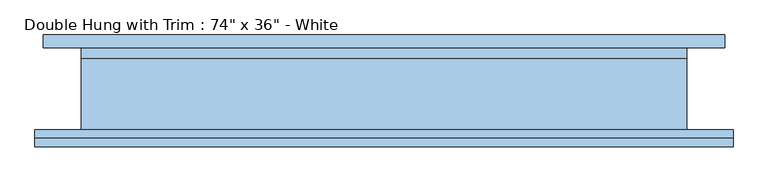
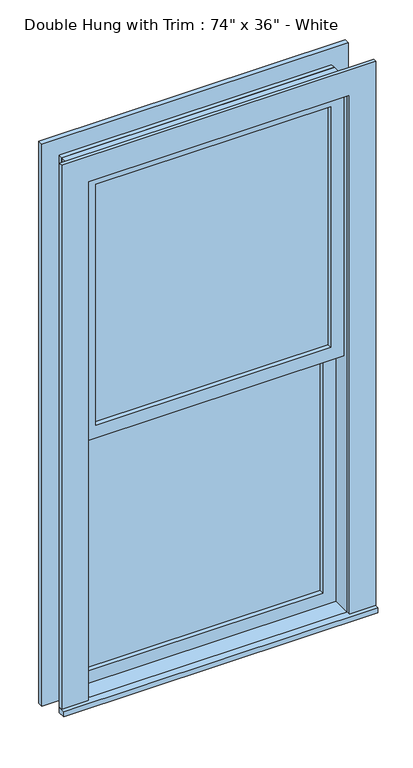
"""IFC4 building model written with IfcOpenShell, lengths in millimetres: window geometry."""

import ifcopenshell
import ifcopenshell.guid

model = None  # the IFC model being written
_history = None  # IfcOwnerHistory: only IFC2X3 demands one
_inside = {}  # id of a spatial element -> (the spatial element, [elements in it])
_under = {}  # id of a project, library or spatial element -> (it, [spatial elements below it])
_declared = {}  # id of a project -> (the project, [libraries it declares])
_typed = {}  # id of a type object -> (the type object, [elements of that type])
_made_of = {}  # id of a material, layer set ... -> (it, [elements and type objects made of it])


def new_model(schema):
    """Start an empty IFC model of exactly this schema.

    Asked for "IFC4X3", IfcOpenShell would pick the latest addendum, in which some entities
    have other attributes; the version numbers below select the first issue.
    IFC2X3 requires an IfcOwnerHistory on every rooted entity: one is made here for all.
    """
    global model, _history
    if schema == "IFC4X3":
        model = ifcopenshell.file(schema_version=(4, 3, 0, 0))
    else:
        model = ifcopenshell.file(schema=schema)
    _inside.clear()
    _under.clear()
    _declared.clear()
    _typed.clear()
    _made_of.clear()
    _history = None
    if model.schema == "IFC2X3":
        org = make("IfcOrganization", Name="unknown")
        user = make(
            "IfcPersonAndOrganization",
            ThePerson=make("IfcPerson", FamilyName="unknown"),
            TheOrganization=org,
        )
        app = make(
            "IfcApplication",
            ApplicationDeveloper=org,
            Version="unknown",
            ApplicationFullName="unknown",
            ApplicationIdentifier="unknown",
        )
        _history = make(
            "IfcOwnerHistory",
            OwningUser=user,
            OwningApplication=app,
            ChangeAction="ADDED",
            CreationDate=0,
        )
    return model


def make(cls, **values):
    """One entity of the class cls with the attributes given. An attribute that is None is left unset."""
    return model.create_entity(
        cls, **{name: value for name, value in values.items() if value is not None}
    )


def rooted(cls, **values):
    """An entity with a GlobalId (a new one), such as an element, a storey or a relation."""
    return make(cls, GlobalId=ifcopenshell.guid.new(), OwnerHistory=_history, **values)


def si_unit(unit_type, name, prefix=None):
    """IfcSIUnit, for example si_unit("LENGTHUNIT", "METRE", prefix="MILLI")."""
    return make("IfcSIUnit", UnitType=unit_type, Prefix=prefix, Name=name)


def assignment(units):
    """IfcUnitAssignment: the units of a project."""
    return None if units is None else make("IfcUnitAssignment", Units=units)


def point(xyz):
    """IfcCartesianPoint."""
    return None if xyz is None else make("IfcCartesianPoint", Coordinates=xyz)


def direction(xyz):
    """IfcDirection."""
    return None if xyz is None else make("IfcDirection", DirectionRatios=xyz)


def frame(location, z_axis=None, x_axis=None):
    """IfcAxis2Placement3D, a coordinate frame: its origin and axes. An axis left out is left unset."""
    return make(
        "IfcAxis2Placement3D",
        Location=point(location),
        Axis=direction(z_axis),
        RefDirection=direction(x_axis),
    )


def origin():
    """The frame at (0, 0, 0) with its axes left unset."""
    return frame((0.0, 0.0, 0.0))


def place(relative_to, where):
    """IfcLocalPlacement: puts the frame where relative to a parent placement (None: the world)."""
    return make(
        "IfcLocalPlacement", PlacementRelTo=relative_to, RelativePlacement=where
    )


def context(
    kind, dimensions, precision=None, world=None, true_north=None, identifier=None
):
    """IfcGeometricRepresentationContext, for example the 3D "Model" context."""
    return make(
        "IfcGeometricRepresentationContext",
        ContextIdentifier=identifier,
        ContextType=kind,
        CoordinateSpaceDimension=dimensions,
        Precision=precision,
        WorldCoordinateSystem=world,
        TrueNorth=true_north,
    )


def project(units=None, contexts=None):
    """IfcProject with its units and contexts."""
    return rooted(
        "IfcProject",
        Name="project",
        RepresentationContexts=contexts,
        UnitsInContext=assignment(units),
    )


def spatial(cls, under=None, at=None, **own):
    """A site, building, storey or space (cls), placed at a placement, below another one or the project."""
    s = rooted(cls, ObjectPlacement=at, **own)
    if under is not None:
        _under.setdefault(under.id(), (under, []))[1].append(s)
    return s


def polyline(points):
    """IfcPolyline through the points."""
    return make("IfcPolyline", Points=[point(p) for p in points])


def outline(outer, holes=None, kind="AREA"):
    """IfcArbitraryClosedProfileDef: a profile drawn as a closed curve; with holes, ...WithVoids."""
    if holes is None:
        return make("IfcArbitraryClosedProfileDef", ProfileType=kind, OuterCurve=outer)
    return make(
        "IfcArbitraryProfileDefWithVoids",
        ProfileType=kind,
        OuterCurve=outer,
        InnerCurves=holes,
    )


def extrude(swept, where, along, depth):
    """IfcExtrudedAreaSolid: the profile swept, set in the frame where, extruded along a direction by depth."""
    return make(
        "IfcExtrudedAreaSolid",
        SweptArea=swept,
        Position=where,
        ExtrudedDirection=direction(along),
        Depth=depth,
    )


def shape(context_of_items, identifier, shape_type, items):
    """IfcShapeRepresentation: the items that make up one representation, for example the "Body"."""
    return make(
        "IfcShapeRepresentation",
        ContextOfItems=context_of_items,
        RepresentationIdentifier=identifier,
        RepresentationType=shape_type,
        Items=items,
    )


def source(mapping_origin, context_of_items, identifier, shape_type, items):
    """IfcRepresentationMap: a shape defined once, which mapped items show again and again."""
    return make(
        "IfcRepresentationMap",
        MappingOrigin=mapping_origin,
        MappedRepresentation=shape(context_of_items, identifier, shape_type, items),
    )


def transform(
    local_origin,
    x_axis=None,
    y_axis=None,
    z_axis=None,
    scale=None,
    scale2=None,
    scale3=None,
    uniform=True,
):
    """IfcCartesianTransformationOperator3D, or its non-uniform kind. x_axis, y_axis, z_axis: its Axis1, 2, 3."""
    if uniform:
        return make(
            "IfcCartesianTransformationOperator3D",
            Axis1=direction(x_axis),
            Axis2=direction(y_axis),
            LocalOrigin=point(local_origin),
            Scale=scale,
            Axis3=direction(z_axis),
        )
    return make(
        "IfcCartesianTransformationOperator3DnonUniform",
        Axis1=direction(x_axis),
        Axis2=direction(y_axis),
        LocalOrigin=point(local_origin),
        Scale=scale,
        Axis3=direction(z_axis),
        Scale2=scale2,
        Scale3=scale3,
    )


def mapped(mapping_source, mapping_target):
    """IfcMappedItem: shows the shape of a source again, moved by a transform."""
    return make(
        "IfcMappedItem", MappingSource=mapping_source, MappingTarget=mapping_target
    )


def made_of(thing, what):
    """Note that an element or type object is made of a material, layer set ...; save() writes the relation."""
    if what is not None:
        _made_of.setdefault(what.id(), (what, []))[1].append(thing)
    return thing


def element(
    cls,
    number,
    at=None,
    inside=None,
    cuts=None,
    type_object=None,
    material=None,
    context=None,
    identifier="Body",
    shape_type=None,
    held_by="IfcProductDefinitionShape",
    body=None,
    shapes=None,
    **own,
):
    """One element of the class cls, such as IfcWall. Its Tag is "e" and its number.

    at: its placement. inside: the storey or other place that contains it. cuts: it is an
    opening in that element (IfcRelVoidsElement). A single representation is given by context,
    identifier, shape_type and body (its items); several are given by shapes. held_by: the class
    of the entity that holds the representations. save() writes the other relations.
    """
    e = rooted(cls, Tag="e%d" % number, ObjectPlacement=at, **own)
    if body is not None:
        shapes = [shape(context, identifier, shape_type, body)]
    if shapes is not None:
        e.Representation = make(held_by, Representations=shapes)
    if inside is not None:
        _inside.setdefault(inside.id(), (inside, []))[1].append(e)
    if cuts is not None:
        rooted(
            "IfcRelVoidsElement", RelatingBuildingElement=cuts, RelatedOpeningElement=e
        )
    if type_object is not None:
        _typed.setdefault(type_object.id(), (type_object, []))[1].append(e)
    return made_of(e, material)


def aggregate(whole, parts):
    """IfcRelAggregates: a whole, such as a stair, and the parts it consists of."""
    return rooted("IfcRelAggregates", RelatingObject=whole, RelatedObjects=parts)


def save(model, path):
    """Write the relations noted so far, then the file.

    IfcRelAggregates (storeys below a building ...), IfcRelContainedInSpatialStructure (elements
    in a storey), IfcRelDefinesByType, IfcRelAssociatesMaterial and IfcRelDeclares: one each for
    every whole, place, type object, material and project.
    """
    for whole, parts in _under.values():
        aggregate(whole, parts)
    for where, things in _inside.values():
        rooted(
            "IfcRelContainedInSpatialStructure",
            RelatedElements=things,
            RelatingStructure=where,
        )
    for kind, things in _typed.values():
        rooted("IfcRelDefinesByType", RelatedObjects=things, RelatingType=kind)
    for what, things in _made_of.values():
        rooted("IfcRelAssociatesMaterial", RelatedObjects=things, RelatingMaterial=what)
    for by, libraries in _declared.values():
        rooted("IfcRelDeclares", RelatingContext=by, RelatedDefinitions=libraries)
    model.write(path)


def window_699487aa(model_context):
    return source(origin(), model_context, "Body", "SweptSolid", [
        extrude(outline(polyline([(-393.7, 17.4625), (-393.7, 30.1625), (393.7, 30.1625), (393.7, 17.4625), (-393.7, 17.4625)])), frame((0.0, 0.0, 571.5), z_axis=(0.0, 0.0, 1.0), x_axis=(1.0, 0.0, 0.0)), (0.0, 0.0, 1.0), 854.075),
        extrude(outline(polyline([(1470.025, -438.15), (527.05, -438.15), (527.05, 438.15), (1470.025, 438.15), (1470.025, -438.15)]), holes=[polyline([(1425.575, -393.7), (1425.575, 393.7), (571.5, 393.7), (571.5, -393.7), (1425.575, -393.7)])]), frame((0.0, 1.5875, 0.0), z_axis=(0.0, 1.0, 0.0), x_axis=(0.0, 0.0, 1.0)), (0.0, 0.0, 1.0), 44.45),
        extrude(outline(polyline([(-527.05, -87.3125), (-527.05, -61.9125), (527.05, -61.9125), (527.05, -87.3125), (-527.05, -87.3125)])), frame((0.0, 0.0, 508.0), z_axis=(0.0, 0.0, 1.0), x_axis=(1.0, 0.0, 0.0)), (0.0, 0.0, 1.0), 19.05),
        extrude(outline(polyline([(2368.55, -438.15), (2368.55, 438.15), (527.05, 438.15), (527.05, 527.05), (2457.45, 527.05), (2457.45, -527.05), (527.05, -527.05), (527.05, -438.15), (2368.55, -438.15)])), frame((0.0, -74.6125, 0.0), z_axis=(0.0, 1.0, 0.0), x_axis=(0.0, 0.0, 1.0)), (0.0, 0.0, 1.0), 12.7),
        extrude(outline(polyline([(2444.75, 514.35), (2444.75, -514.35), (450.85, -514.35), (450.85, 514.35), (2444.75, 514.35)]), holes=[polyline([(2355.85, 425.45), (539.75, 425.45), (539.75, -425.45), (2355.85, -425.45), (2355.85, 425.45)])]), frame((0.0, 61.9125, 0.0), z_axis=(0.0, 1.0, 0.0), x_axis=(0.0, 0.0, 1.0)), (0.0, 0.0, 1.0), 19.05),
        extrude(outline(polyline([(393.7, -14.2875), (393.7, -26.9875), (-393.7, -26.9875), (-393.7, -14.2875), (393.7, -14.2875)])), frame((0.0, 0.0, 1470.025), z_axis=(0.0, 0.0, 1.0), x_axis=(1.0, 0.0, 0.0)), (0.0, 0.0, 1.0), 854.075),
        extrude(outline(polyline([(2368.55, -438.15), (1425.575, -438.15), (1425.575, 438.15), (2368.55, 438.15), (2368.55, -438.15)]), holes=[polyline([(2324.1, -393.7), (2324.1, 393.7), (1470.025, 393.7), (1470.025, -393.7), (2324.1, -393.7)])]), frame((0.0, -42.8625, 0.0), z_axis=(0.0, 1.0, 0.0), x_axis=(0.0, 0.0, 1.0)), (0.0, 0.0, 1.0), 44.45),
        extrude(outline(polyline([(2387.6, -457.2), (508.0, -457.2), (508.0, 457.2), (2387.6, 457.2), (2387.6, -457.2)]), holes=[polyline([(2355.85, -425.45), (2355.85, 425.45), (539.75, 425.45), (539.75, -425.45), (2355.85, -425.45)])]), frame((0.0, 46.0375, 0.0), z_axis=(0.0, 1.0, 0.0), x_axis=(0.0, 0.0, 1.0)), (0.0, 0.0, 1.0), 15.875),
        extrude(outline(polyline([(2387.6, 457.2), (2387.6, -457.2), (508.0, -457.2), (508.0, 457.2), (2387.6, 457.2)]), holes=[polyline([(2368.55, 438.15), (527.05, 438.15), (527.05, -438.15), (2368.55, -438.15), (2368.55, 438.15)])]), frame((0.0, -61.9125, 0.0), z_axis=(0.0, 1.0, 0.0), x_axis=(0.0, 0.0, 1.0)), (0.0, 0.0, 1.0), 107.95),
    ])


if __name__ == "__main__":
    model = new_model("IFC4")
    model_context = context("Model", 3, world=origin())
    ifc_project = project(units=[si_unit("LENGTHUNIT", "METRE", prefix="MILLI")], contexts=[model_context])
    site = spatial("IfcSite", under=ifc_project)
    building = spatial("IfcBuilding", under=site)
    placement = place(None, origin())
    window_shape = window_699487aa(model_context)
    element("IfcWindow", 1, ObjectType="Double Hung with Trim : 74\" x 36\" - White", at=placement, inside=building, context=model_context, shape_type="MappedRepresentation", body=[
        mapped(window_shape, transform((0.0, 0.0, 0.0), x_axis=(1.0, 0.0, 0.0), y_axis=(0.0, 1.0, 0.0), z_axis=(0.0, 0.0, 1.0))),
    ])
    save(model, "model.ifc")

# Revit data of these elements
# Type "Double Hung with Trim : 74\" x 36\" - White"
#   Type Mark = "23"
#   COBie.Type.CreatedBy = "doug.wood@us.ibm.com"
#   COBie.Type.CreatedOn = "2016-04-14T02:07:26"
#   COBie.Type.Name = "Windows_Double Hung with Trim_74\" x 36\"_23"
#   COBie.Type.Category = "23-30 20 17 17 14 : Double-Hung Windows"
#   COBie.Type.Description = "Double Hung with Trim_74\" x 36\""
#   COBie.Type.Manufacturer = ""
#   COBie.Type.ModelNumber = ""
#   Construction Type Id = "GSP4R"
#   Assembly Code = "B2020100"
#   Analytic Construction = "1/8 in Pilkington single glazing"
#   COBie.Type.ReplacementCost = 0
#   Visual Light Transmittance = 0.9
#   Solar Heat Gain Coefficient = 0.78
#   Heat Transfer Coefficient (U) = 3.6886 W/(m²·K)
#   Height = 6' - 2"
#   Default Sill Height = 1' - 8"
#   Trim Projection - Ext. = 0' - 0 1/2"
#   Trim Projection - Int. = 0' - 0 3/4"
#   Trim Width - Exterior = 0' - 3 1/2"
#   Trim Width - Interior = 0' - 3 1/2"
#   Width = 3' - 0"
#   Window Inset = 0' - 0 3/4"
#   COBie.Type = no
#   Glass Pane Material = Glass
#   Sash Material = Sash - White
#   Trim Exterior Material = Trim - White
#   Trim Interior Material = Trim - White
#   Wall Closure = (empty or 0)
# Element 1 (IfcWindow, "Double Hung with Trim : 74\" x 36\" - White")
#   Materials on its faces: "Sash - White", "Trim - White", "Glass"
# Materials
#   "Glass": class "Glass", colour RGB 0 128 192, transparency 0.75, Description = "Soda Lime Glass", Cost = 0
#   "Sash - White": class "Wood", colour RGB 255 255 255, transparency 0, Cost = 0
#   "Trim - White": class "Wood", colour RGB 255 255 255, transparency 0, Cost = 0
